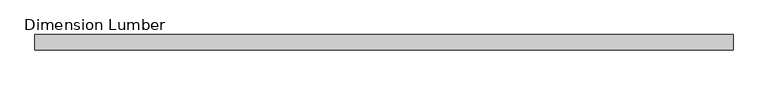
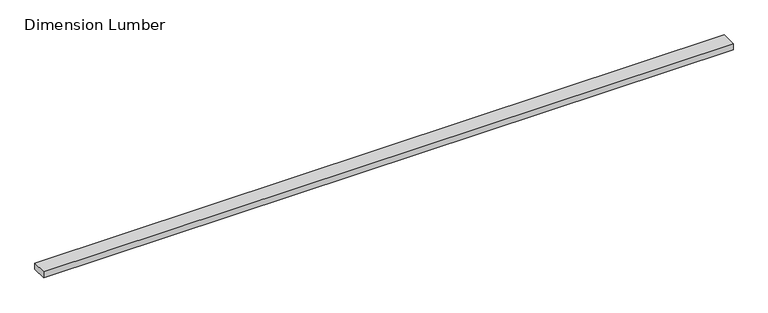
"""IFC4 building model written with IfcOpenShell, lengths in millimetres: beam geometry, Dimension Lumber : Top Supporting Lumbers."""

from ifc_helpers import new_model, si_unit, frame, origin, place, context, project, spatial, polyline, outline, extrude, source, transform, mapped, element, save


def dimension_lumber_22ea9708(model_context):
    return source(origin(), model_context, "Body", "SweptSolid", [
        extrude(outline(polyline([(2035.175, 44.45), (2035.175, -44.45), (-2035.175, -44.45), (-2035.175, 44.45), (2035.175, 44.45)])), frame((0.0, 0.0, -19.05), z_axis=(0.0, 0.0, 1.0), x_axis=(1.0, 0.0, 0.0)), (0.0, 0.0, 1.0), 38.1),
    ])


if __name__ == "__main__":
    model = new_model("IFC4")
    model_context = context("Model", 3, world=origin())
    ifc_project = project(units=[si_unit("LENGTHUNIT", "METRE", prefix="MILLI")], contexts=[model_context])
    site = spatial("IfcSite", under=ifc_project)
    building = spatial("IfcBuilding", under=site)
    placement = place(None, origin())
    dimension_lumber_shape = dimension_lumber_22ea9708(model_context)
    element("IfcBeam", 1, ObjectType="Dimension Lumber : Top Supporting Lumbers", at=placement, inside=building, context=model_context, shape_type="MappedRepresentation", body=[
        mapped(dimension_lumber_shape, transform((0.0, 0.0, 0.0), x_axis=(1.0, 0.0, 0.0), y_axis=(0.0, 1.0, 0.0), z_axis=(0.0, 0.0, 1.0))),
    ])
    save(model, "model.ifc")

# Revit data of these elements
# Type "Dimension Lumber : Top Supporting Lumbers"
#   Assembly Code = "B10"
#   A = 0.0364583 SF
#   Length [instance default] = 5' - 0"
#   b = 0' - 3 1/2"
#   d = 0' - 1 1/2"
#   Structural Material [instance default] = Softwood, Lumber
# Element 1 (IfcBeam, "Dimension Lumber : Top Supporting Lumbers")
#   Structural Material = Douglas Fir #2
#   Materials on its faces: "Douglas Fir #2"
# Materials
#   "Softwood, Lumber": class "Wood", colour RGB 223 192 134, transparency 0, Description = "Pinus Echinata", Cost = 0
#   "Douglas Fir #2": class "Wood", colour RGB 223 192 134, transparency 0, Description = "Pinus Echinata", Cost = 0
